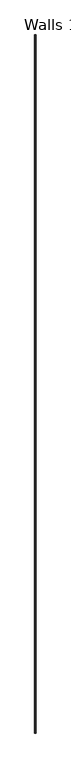
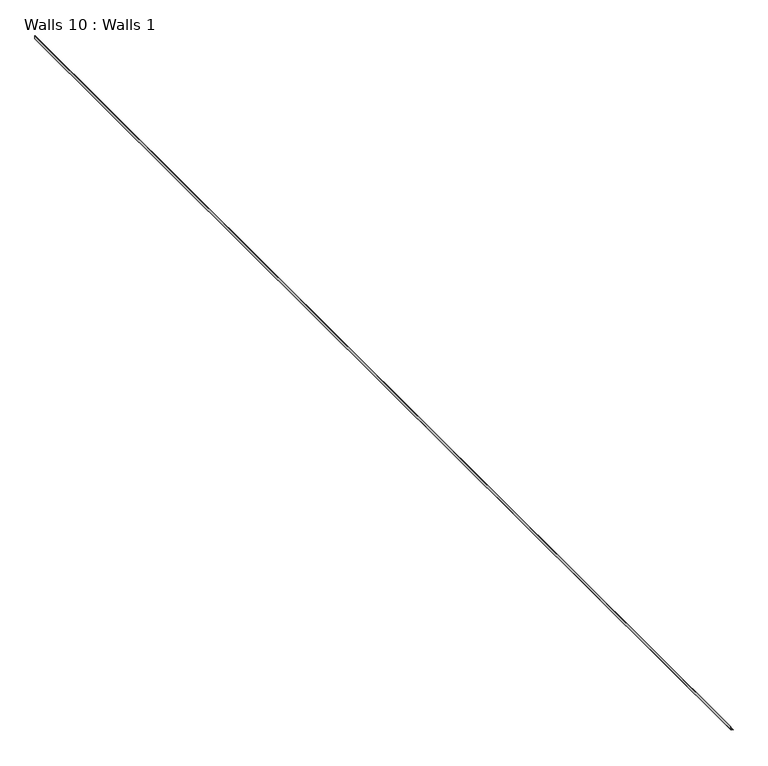
"""IFC4 building model written with IfcOpenShell, lengths in millimetres: proxy geometry, Walls 10 : Walls 1."""

import ifcopenshell
import ifcopenshell.guid

model = None  # the IFC model being written
_history = None  # IfcOwnerHistory: only IFC2X3 demands one
_inside = {}  # id of a spatial element -> (the spatial element, [elements in it])
_under = {}  # id of a project, library or spatial element -> (it, [spatial elements below it])
_declared = {}  # id of a project -> (the project, [libraries it declares])
_typed = {}  # id of a type object -> (the type object, [elements of that type])
_made_of = {}  # id of a material, layer set ... -> (it, [elements and type objects made of it])


def new_model(schema):
    """Start an empty IFC model of exactly this schema.

    Asked for "IFC4X3", IfcOpenShell would pick the latest addendum, in which some entities
    have other attributes; the version numbers below select the first issue.
    IFC2X3 requires an IfcOwnerHistory on every rooted entity: one is made here for all.
    """
    global model, _history
    if schema == "IFC4X3":
        model = ifcopenshell.file(schema_version=(4, 3, 0, 0))
    else:
        model = ifcopenshell.file(schema=schema)
    _inside.clear()
    _under.clear()
    _declared.clear()
    _typed.clear()
    _made_of.clear()
    _history = None
    if model.schema == "IFC2X3":
        org = make("IfcOrganization", Name="unknown")
        user = make(
            "IfcPersonAndOrganization",
            ThePerson=make("IfcPerson", FamilyName="unknown"),
            TheOrganization=org,
        )
        app = make(
            "IfcApplication",
            ApplicationDeveloper=org,
            Version="unknown",
            ApplicationFullName="unknown",
            ApplicationIdentifier="unknown",
        )
        _history = make(
            "IfcOwnerHistory",
            OwningUser=user,
            OwningApplication=app,
            ChangeAction="ADDED",
            CreationDate=0,
        )
    return model


def make(cls, **values):
    """One entity of the class cls with the attributes given. An attribute that is None is left unset."""
    return model.create_entity(
        cls, **{name: value for name, value in values.items() if value is not None}
    )


def rooted(cls, **values):
    """An entity with a GlobalId (a new one), such as an element, a storey or a relation."""
    return make(cls, GlobalId=ifcopenshell.guid.new(), OwnerHistory=_history, **values)


def si_unit(unit_type, name, prefix=None):
    """IfcSIUnit, for example si_unit("LENGTHUNIT", "METRE", prefix="MILLI")."""
    return make("IfcSIUnit", UnitType=unit_type, Prefix=prefix, Name=name)


def assignment(units):
    """IfcUnitAssignment: the units of a project."""
    return None if units is None else make("IfcUnitAssignment", Units=units)


def point(xyz):
    """IfcCartesianPoint."""
    return None if xyz is None else make("IfcCartesianPoint", Coordinates=xyz)


def direction(xyz):
    """IfcDirection."""
    return None if xyz is None else make("IfcDirection", DirectionRatios=xyz)


def frame(location, z_axis=None, x_axis=None):
    """IfcAxis2Placement3D, a coordinate frame: its origin and axes. An axis left out is left unset."""
    return make(
        "IfcAxis2Placement3D",
        Location=point(location),
        Axis=direction(z_axis),
        RefDirection=direction(x_axis),
    )


def origin():
    """The frame at (0, 0, 0) with its axes left unset."""
    return frame((0.0, 0.0, 0.0))


def place(relative_to, where):
    """IfcLocalPlacement: puts the frame where relative to a parent placement (None: the world)."""
    return make(
        "IfcLocalPlacement", PlacementRelTo=relative_to, RelativePlacement=where
    )


def context(
    kind, dimensions, precision=None, world=None, true_north=None, identifier=None
):
    """IfcGeometricRepresentationContext, for example the 3D "Model" context."""
    return make(
        "IfcGeometricRepresentationContext",
        ContextIdentifier=identifier,
        ContextType=kind,
        CoordinateSpaceDimension=dimensions,
        Precision=precision,
        WorldCoordinateSystem=world,
        TrueNorth=true_north,
    )


def project(units=None, contexts=None):
    """IfcProject with its units and contexts."""
    return rooted(
        "IfcProject",
        Name="project",
        RepresentationContexts=contexts,
        UnitsInContext=assignment(units),
    )


def spatial(cls, under=None, at=None, **own):
    """A site, building, storey or space (cls), placed at a placement, below another one or the project."""
    s = rooted(cls, ObjectPlacement=at, **own)
    if under is not None:
        _under.setdefault(under.id(), (under, []))[1].append(s)
    return s


def polyline(points):
    """IfcPolyline through the points."""
    return make("IfcPolyline", Points=[point(p) for p in points])


def outline(outer, holes=None, kind="AREA"):
    """IfcArbitraryClosedProfileDef: a profile drawn as a closed curve; with holes, ...WithVoids."""
    if holes is None:
        return make("IfcArbitraryClosedProfileDef", ProfileType=kind, OuterCurve=outer)
    return make(
        "IfcArbitraryProfileDefWithVoids",
        ProfileType=kind,
        OuterCurve=outer,
        InnerCurves=holes,
    )


def extrude(swept, where, along, depth):
    """IfcExtrudedAreaSolid: the profile swept, set in the frame where, extruded along a direction by depth."""
    return make(
        "IfcExtrudedAreaSolid",
        SweptArea=swept,
        Position=where,
        ExtrudedDirection=direction(along),
        Depth=depth,
    )


def shape(context_of_items, identifier, shape_type, items):
    """IfcShapeRepresentation: the items that make up one representation, for example the "Body"."""
    return make(
        "IfcShapeRepresentation",
        ContextOfItems=context_of_items,
        RepresentationIdentifier=identifier,
        RepresentationType=shape_type,
        Items=items,
    )


def source(mapping_origin, context_of_items, identifier, shape_type, items):
    """IfcRepresentationMap: a shape defined once, which mapped items show again and again."""
    return make(
        "IfcRepresentationMap",
        MappingOrigin=mapping_origin,
        MappedRepresentation=shape(context_of_items, identifier, shape_type, items),
    )


def transform(
    local_origin,
    x_axis=None,
    y_axis=None,
    z_axis=None,
    scale=None,
    scale2=None,
    scale3=None,
    uniform=True,
):
    """IfcCartesianTransformationOperator3D, or its non-uniform kind. x_axis, y_axis, z_axis: its Axis1, 2, 3."""
    if uniform:
        return make(
            "IfcCartesianTransformationOperator3D",
            Axis1=direction(x_axis),
            Axis2=direction(y_axis),
            LocalOrigin=point(local_origin),
            Scale=scale,
            Axis3=direction(z_axis),
        )
    return make(
        "IfcCartesianTransformationOperator3DnonUniform",
        Axis1=direction(x_axis),
        Axis2=direction(y_axis),
        LocalOrigin=point(local_origin),
        Scale=scale,
        Axis3=direction(z_axis),
        Scale2=scale2,
        Scale3=scale3,
    )


def mapped(mapping_source, mapping_target):
    """IfcMappedItem: shows the shape of a source again, moved by a transform."""
    return make(
        "IfcMappedItem", MappingSource=mapping_source, MappingTarget=mapping_target
    )


def made_of(thing, what):
    """Note that an element or type object is made of a material, layer set ...; save() writes the relation."""
    if what is not None:
        _made_of.setdefault(what.id(), (what, []))[1].append(thing)
    return thing


def element(
    cls,
    number,
    at=None,
    inside=None,
    cuts=None,
    type_object=None,
    material=None,
    context=None,
    identifier="Body",
    shape_type=None,
    held_by="IfcProductDefinitionShape",
    body=None,
    shapes=None,
    **own,
):
    """One element of the class cls, such as IfcWall. Its Tag is "e" and its number.

    at: its placement. inside: the storey or other place that contains it. cuts: it is an
    opening in that element (IfcRelVoidsElement). A single representation is given by context,
    identifier, shape_type and body (its items); several are given by shapes. held_by: the class
    of the entity that holds the representations. save() writes the other relations.
    """
    e = rooted(cls, Tag="e%d" % number, ObjectPlacement=at, **own)
    if body is not None:
        shapes = [shape(context, identifier, shape_type, body)]
    if shapes is not None:
        e.Representation = make(held_by, Representations=shapes)
    if inside is not None:
        _inside.setdefault(inside.id(), (inside, []))[1].append(e)
    if cuts is not None:
        rooted(
            "IfcRelVoidsElement", RelatingBuildingElement=cuts, RelatedOpeningElement=e
        )
    if type_object is not None:
        _typed.setdefault(type_object.id(), (type_object, []))[1].append(e)
    return made_of(e, material)


def aggregate(whole, parts):
    """IfcRelAggregates: a whole, such as a stair, and the parts it consists of."""
    return rooted("IfcRelAggregates", RelatingObject=whole, RelatedObjects=parts)


def save(model, path):
    """Write the relations noted so far, then the file.

    IfcRelAggregates (storeys below a building ...), IfcRelContainedInSpatialStructure (elements
    in a storey), IfcRelDefinesByType, IfcRelAssociatesMaterial and IfcRelDeclares: one each for
    every whole, place, type object, material and project.
    """
    for whole, parts in _under.values():
        aggregate(whole, parts)
    for where, things in _inside.values():
        rooted(
            "IfcRelContainedInSpatialStructure",
            RelatedElements=things,
            RelatingStructure=where,
        )
    for kind, things in _typed.values():
        rooted("IfcRelDefinesByType", RelatedObjects=things, RelatingType=kind)
    for what, things in _made_of.values():
        rooted("IfcRelAssociatesMaterial", RelatedObjects=things, RelatingMaterial=what)
    for by, libraries in _declared.values():
        rooted("IfcRelDeclares", RelatingContext=by, RelatedDefinitions=libraries)
    model.write(path)


def walls_10_walls_1_a2aab447(model_context):
    return source(origin(), model_context, "Body", "SweptSolid", [
        extrude(outline(polyline([(271905.9525271, 32173.0125149), (271907.0750591, 32174.1350469), (271914.7780545, 32166.4320516), (271914.7780545, 32154.4122028), (271941.9369568, 32154.4122028), (271941.9369568, 32152.8247028), (271913.1905545, 32152.8247028), (271913.1905545, 32165.7744875), (271905.9525271, 32173.0125149)])), frame((0.0, 29659.1292286, 0.0), z_axis=(0.0, 1.0, 0.0), x_axis=(0.0, 0.0, 1.0)), (0.0, 0.0, 1.0), 11114.5564326),
    ])


if __name__ == "__main__":
    model = new_model("IFC4")
    model_context = context("Model", 3, world=origin())
    ifc_project = project(units=[si_unit("LENGTHUNIT", "METRE", prefix="MILLI")], contexts=[model_context])
    site = spatial("IfcSite", under=ifc_project)
    building = spatial("IfcBuilding", under=site)
    placement = place(None, origin())
    walls_10_walls_1_shape = walls_10_walls_1_a2aab447(model_context)
    element("IfcBuildingElementProxy", 1, Name="Walls 10 : Walls 1", ObjectType="Walls 10 : Walls 1", at=placement, inside=building, context=model_context, shape_type="MappedRepresentation", body=[
        mapped(walls_10_walls_1_shape, transform((0.0, 0.0, 0.0), x_axis=(1.0, 0.0, 0.0), y_axis=(0.0, 1.0, 0.0), z_axis=(0.0, 0.0, 1.0))),
    ])
    save(model, "model.ifc")

# Revit data of these elements
# Element 1 (IfcBuildingElementProxy, "Walls 10 : Walls 1")
#   Materials on its faces: "GALV. BRAKE METAL - (COLOR: MATCH ALUM. WINDOWS)"
# Materials
#   "GALV. BRAKE METAL - (COLOR: MATCH ALUM. WINDOWS)": class "Generic", colour RGB 234 234 234, transparency 0, Cost = 0
